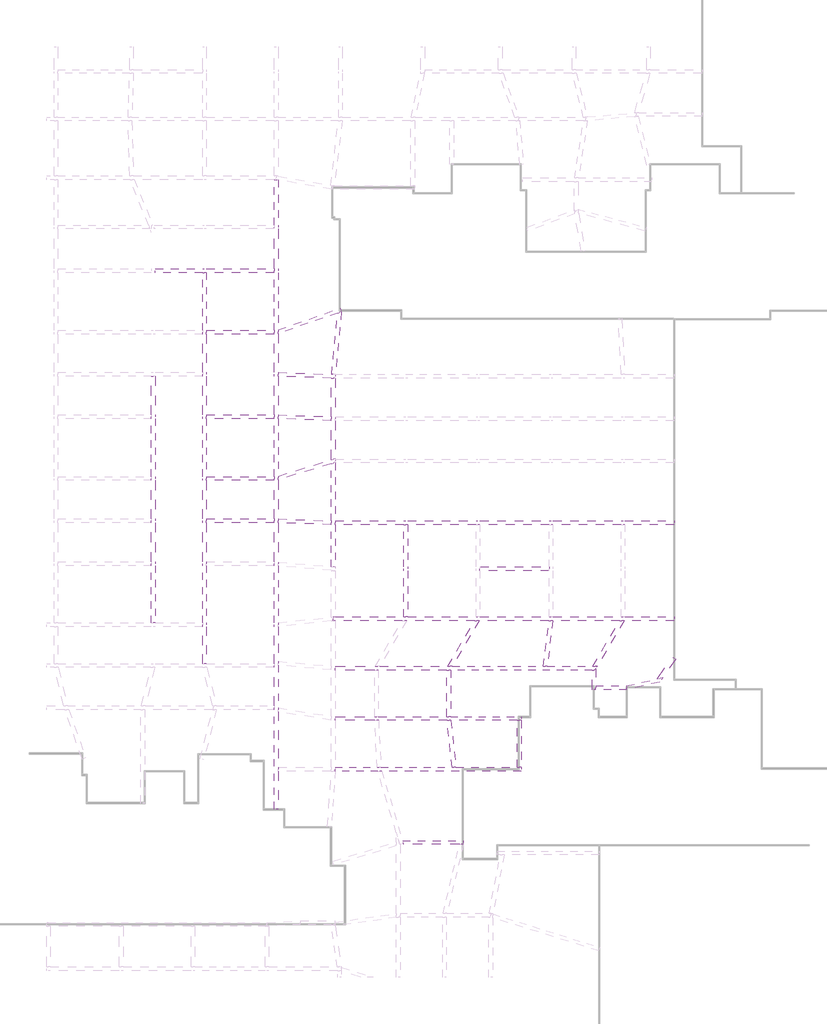
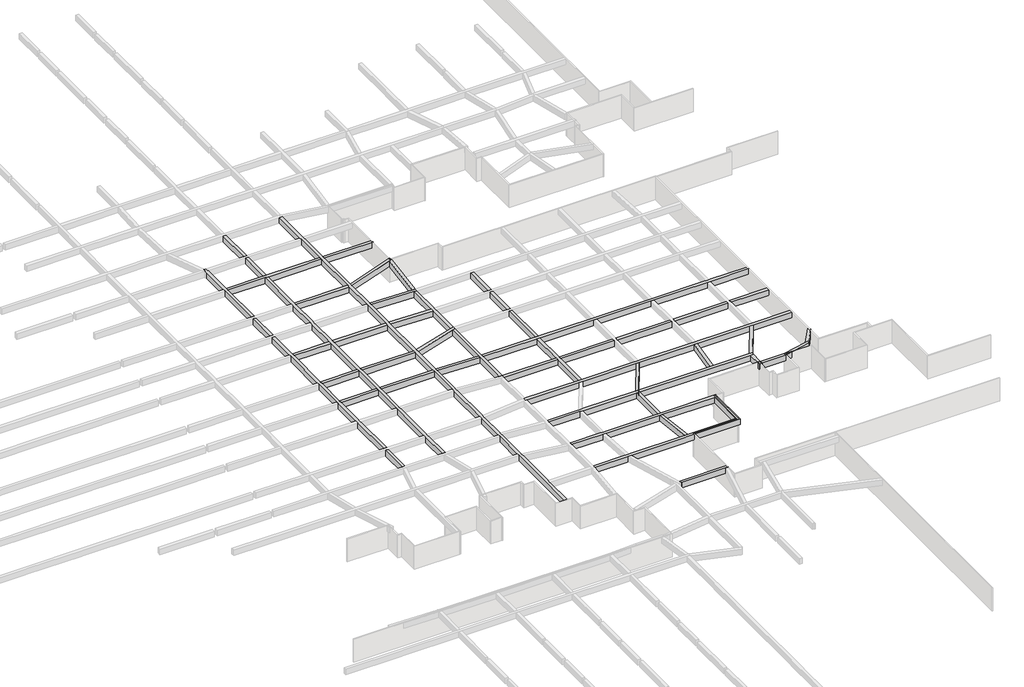
# One storey, part 42 of 45: 34 beams.
"""IFC4 building model written with IfcOpenShell, lengths in millimetres."""

import ifcopenshell
import ifcopenshell.guid

model = None  # the IFC model being written
_history = None  # IfcOwnerHistory: only IFC2X3 demands one
_inside = {}  # id of a spatial element -> (the spatial element, [elements in it])
_under = {}  # id of a project, library or spatial element -> (it, [spatial elements below it])
_declared = {}  # id of a project -> (the project, [libraries it declares])
_typed = {}  # id of a type object -> (the type object, [elements of that type])
_made_of = {}  # id of a material, layer set ... -> (it, [elements and type objects made of it])


def new_model(schema):
    """Start an empty IFC model of exactly this schema.

    Asked for "IFC4X3", IfcOpenShell would pick the latest addendum, in which some entities
    have other attributes; the version numbers below select the first issue.
    IFC2X3 requires an IfcOwnerHistory on every rooted entity: one is made here for all.
    """
    global model, _history
    if schema == "IFC4X3":
        model = ifcopenshell.file(schema_version=(4, 3, 0, 0))
    else:
        model = ifcopenshell.file(schema=schema)
    _inside.clear()
    _under.clear()
    _declared.clear()
    _typed.clear()
    _made_of.clear()
    _history = None
    if model.schema == "IFC2X3":
        org = make("IfcOrganization", Name="unknown")
        user = make(
            "IfcPersonAndOrganization",
            ThePerson=make("IfcPerson", FamilyName="unknown"),
            TheOrganization=org,
        )
        app = make(
            "IfcApplication",
            ApplicationDeveloper=org,
            Version="unknown",
            ApplicationFullName="unknown",
            ApplicationIdentifier="unknown",
        )
        _history = make(
            "IfcOwnerHistory",
            OwningUser=user,
            OwningApplication=app,
            ChangeAction="ADDED",
            CreationDate=0,
        )
    return model


def make(cls, **values):
    """One entity of the class cls with the attributes given. An attribute that is None is left unset."""
    return model.create_entity(
        cls, **{name: value for name, value in values.items() if value is not None}
    )


def rooted(cls, **values):
    """An entity with a GlobalId (a new one), such as an element, a storey or a relation."""
    return make(cls, GlobalId=ifcopenshell.guid.new(), OwnerHistory=_history, **values)


def si_unit(unit_type, name, prefix=None):
    """IfcSIUnit, for example si_unit("LENGTHUNIT", "METRE", prefix="MILLI")."""
    return make("IfcSIUnit", UnitType=unit_type, Prefix=prefix, Name=name)


def assignment(units):
    """IfcUnitAssignment: the units of a project."""
    return None if units is None else make("IfcUnitAssignment", Units=units)


def point(xyz):
    """IfcCartesianPoint."""
    return None if xyz is None else make("IfcCartesianPoint", Coordinates=xyz)


def direction(xyz):
    """IfcDirection."""
    return None if xyz is None else make("IfcDirection", DirectionRatios=xyz)


def frame(location, z_axis=None, x_axis=None):
    """IfcAxis2Placement3D, a coordinate frame: its origin and axes. An axis left out is left unset."""
    return make(
        "IfcAxis2Placement3D",
        Location=point(location),
        Axis=direction(z_axis),
        RefDirection=direction(x_axis),
    )


def origin():
    """The frame at (0, 0, 0) with its axes left unset."""
    return frame((0.0, 0.0, 0.0))


def place(relative_to, where):
    """IfcLocalPlacement: puts the frame where relative to a parent placement (None: the world)."""
    return make(
        "IfcLocalPlacement", PlacementRelTo=relative_to, RelativePlacement=where
    )


def context(
    kind, dimensions, precision=None, world=None, true_north=None, identifier=None
):
    """IfcGeometricRepresentationContext, for example the 3D "Model" context."""
    return make(
        "IfcGeometricRepresentationContext",
        ContextIdentifier=identifier,
        ContextType=kind,
        CoordinateSpaceDimension=dimensions,
        Precision=precision,
        WorldCoordinateSystem=world,
        TrueNorth=true_north,
    )


def project(units=None, contexts=None):
    """IfcProject with its units and contexts."""
    return rooted(
        "IfcProject",
        Name="project",
        RepresentationContexts=contexts,
        UnitsInContext=assignment(units),
    )


def spatial(cls, under=None, at=None, **own):
    """A site, building, storey or space (cls), placed at a placement, below another one or the project."""
    s = rooted(cls, ObjectPlacement=at, **own)
    if under is not None:
        _under.setdefault(under.id(), (under, []))[1].append(s)
    return s


def polyline(points):
    """IfcPolyline through the points."""
    return make("IfcPolyline", Points=[point(p) for p in points])


def outline(outer, holes=None, kind="AREA"):
    """IfcArbitraryClosedProfileDef: a profile drawn as a closed curve; with holes, ...WithVoids."""
    if holes is None:
        return make("IfcArbitraryClosedProfileDef", ProfileType=kind, OuterCurve=outer)
    return make(
        "IfcArbitraryProfileDefWithVoids",
        ProfileType=kind,
        OuterCurve=outer,
        InnerCurves=holes,
    )


def extrude(swept, where, along, depth):
    """IfcExtrudedAreaSolid: the profile swept, set in the frame where, extruded along a direction by depth."""
    return make(
        "IfcExtrudedAreaSolid",
        SweptArea=swept,
        Position=where,
        ExtrudedDirection=direction(along),
        Depth=depth,
    )


def faces_of(points, faces, orient=None, outer=None):
    """IfcFace entities. A face is a list of loops; a loop is a list of indices into points, from 0.

    orient and outer hold one flag for each loop. By default every Orientation is true, the
    first loop of a face is its IfcFaceOuterBound and the others are IfcFaceBound.
    """
    made = []
    for i, loops in enumerate(faces):
        bounds = []
        for j, loop in enumerate(loops):
            is_outer = j == 0 if outer is None else outer[i][j]
            bounds.append(
                make(
                    "IfcFaceOuterBound" if is_outer else "IfcFaceBound",
                    Bound=make("IfcPolyLoop", Polygon=[points[k] for k in loop]),
                    Orientation=True if orient is None else orient[i][j],
                )
            )
        made.append(make("IfcFace", Bounds=bounds))
    return made


def faceted_brep(points, faces, orient=None, outer=None, voids=None):
    """IfcFacetedBrep: a solid bounded by flat faces; with voids (closed shells), ...WithVoids."""
    shared = [point(p) for p in points]
    hull = make("IfcClosedShell", CfsFaces=faces_of(shared, faces, orient, outer))
    if voids is None:
        return make("IfcFacetedBrep", Outer=hull)
    return make(
        "IfcFacetedBrepWithVoids",
        Outer=hull,
        Voids=[
            make(cls, CfsFaces=faces_of(shared, fs, o, b)) for cls, fs, o, b in voids
        ],
    )


def shape(context_of_items, identifier, shape_type, items):
    """IfcShapeRepresentation: the items that make up one representation, for example the "Body"."""
    return make(
        "IfcShapeRepresentation",
        ContextOfItems=context_of_items,
        RepresentationIdentifier=identifier,
        RepresentationType=shape_type,
        Items=items,
    )


def made_of(thing, what):
    """Note that an element or type object is made of a material, layer set ...; save() writes the relation."""
    if what is not None:
        _made_of.setdefault(what.id(), (what, []))[1].append(thing)
    return thing


def element(
    cls,
    number,
    at=None,
    inside=None,
    cuts=None,
    type_object=None,
    material=None,
    context=None,
    identifier="Body",
    shape_type=None,
    held_by="IfcProductDefinitionShape",
    body=None,
    shapes=None,
    **own,
):
    """One element of the class cls, such as IfcWall. Its Tag is "e" and its number.

    at: its placement. inside: the storey or other place that contains it. cuts: it is an
    opening in that element (IfcRelVoidsElement). A single representation is given by context,
    identifier, shape_type and body (its items); several are given by shapes. held_by: the class
    of the entity that holds the representations. save() writes the other relations.
    """
    e = rooted(cls, Tag="e%d" % number, ObjectPlacement=at, **own)
    if body is not None:
        shapes = [shape(context, identifier, shape_type, body)]
    if shapes is not None:
        e.Representation = make(held_by, Representations=shapes)
    if inside is not None:
        _inside.setdefault(inside.id(), (inside, []))[1].append(e)
    if cuts is not None:
        rooted(
            "IfcRelVoidsElement", RelatingBuildingElement=cuts, RelatedOpeningElement=e
        )
    if type_object is not None:
        _typed.setdefault(type_object.id(), (type_object, []))[1].append(e)
    return made_of(e, material)


def aggregate(whole, parts):
    """IfcRelAggregates: a whole, such as a stair, and the parts it consists of."""
    return rooted("IfcRelAggregates", RelatingObject=whole, RelatedObjects=parts)


def save(model, path):
    """Write the relations noted so far, then the file.

    IfcRelAggregates (storeys below a building ...), IfcRelContainedInSpatialStructure (elements
    in a storey), IfcRelDefinesByType, IfcRelAssociatesMaterial and IfcRelDeclares: one each for
    every whole, place, type object, material and project.
    """
    for whole, parts in _under.values():
        aggregate(whole, parts)
    for where, things in _inside.values():
        rooted(
            "IfcRelContainedInSpatialStructure",
            RelatedElements=things,
            RelatingStructure=where,
        )
    for kind, things in _typed.values():
        rooted("IfcRelDefinesByType", RelatedObjects=things, RelatingType=kind)
    for what, things in _made_of.values():
        rooted("IfcRelAssociatesMaterial", RelatedObjects=things, RelatingMaterial=what)
    for by, libraries in _declared.values():
        rooted("IfcRelDeclares", RelatingContext=by, RelatedDefinitions=libraries)
    model.write(path)


model = new_model("IFC4")

# Units and contexts
model_context = context("Model", 3, world=origin())
ifc_project = project(units=[si_unit("LENGTHUNIT", "METRE", prefix="MILLI")], contexts=[model_context])

# Site, building, storey
site = spatial("IfcSite", under=ifc_project)
building = spatial("IfcBuilding", under=site)
storey = spatial("IfcBuildingStorey", under=building, Name="户型图", Elevation=0.0)

# Beams
placement = place(None, origin())
element("IfcBeam", 1, ObjectType="混凝土 - 矩形梁 : KL_beam", at=placement, inside=storey, context=model_context, shape_type="Brep", body=[
    faceted_brep([(18058.0309094, 68422.9728882, 3300.0), (17658.0309094, 68422.9728882, 3300.0), (17658.0309094, 68422.9728882, 2500.0), (18058.0309094, 68422.9728882, 2500.0), (18058.0309094, 72491.389713, 3300.0), (18058.0309094, 72891.389713, 3300.0), (18058.0309094, 78847.1860391, 3300.0), (18058.0309094, 79252.1720894, 3300.0), (18058.0309094, 83829.2308834, 3300.0), (18058.0309094, 84230.7588184, 3300.0), (18058.0309094, 87967.4136101, 3300.0), (18058.0309094, 88369.6169219, 3300.0), (18058.0309094, 94470.4509181, 3300.0), (18058.0309094, 94871.9788531, 3300.0), (18058.0309094, 99081.6059995, 3300.0), (18058.0309094, 99481.8498172, 3300.0), (18058.0309094, 103663.2536994, 3300.0), (18058.0309094, 104081.530402, 3300.0), (18058.0309094, 110222.8260342, 3300.0), (18058.0309094, 110623.0698519, 3300.0), (18058.0309094, 114764.7475323, 3300.0), (18058.0309094, 115164.99135, 3300.0), (18058.0309094, 119319.9005194, 3300.0), (18058.0309094, 119742.9487918, 3300.0), (18058.0309094, 125862.5591329, 3300.0), (18058.0309094, 126262.5591329, 3300.0), (18058.0309094, 130536.5288825, 3300.0), (18058.0309094, 130936.5288825, 3300.0), (18058.0309094, 135784.6345106, 3300.0), (17840.6731553, 135822.9605472, 3300.0), (17658.0309094, 135822.9605472, 3300.0), (17658.0309094, 130936.5288825, 3300.0), (17658.0309094, 130536.5288825, 3300.0), (17658.0309094, 126262.5591329, 3300.0), (17658.0309094, 125862.5591329, 3300.0), (17658.0309094, 119662.5591329, 3300.0), (17658.0309094, 119262.5591329, 3300.0), (17658.0309094, 115171.853595, 3300.0), (17658.0309094, 114771.853595, 3300.0), (17658.0309094, 110629.932653, 3300.0), (17658.0309094, 110229.932653, 3300.0), (17658.0309094, 104011.2459144, 3300.0), (17658.0309094, 103611.2459144, 3300.0), (17658.0309094, 99488.7126183, 3300.0), (17658.0309094, 99088.7126183, 3300.0), (17658.0309094, 94888.7126183, 3300.0), (17658.0309094, 94488.7126183, 3300.0), (17658.0309094, 88347.4925836, 3300.0), (17658.0309094, 87947.4925836, 3300.0), (17658.0309094, 83990.1370817, 3300.0), (17658.0309094, 83590.1370817, 3300.0), (17658.0309094, 79472.5341829, 3300.0), (17658.0309094, 79072.5341829, 3300.0), (17658.0309094, 135822.9605472, 2500.0), (17658.0309094, 130936.5288825, 2500.0), (17658.0309094, 130536.5288825, 2500.0), (17658.0309094, 126262.5591329, 2500.0), (17658.0309094, 125862.5591329, 2500.0), (17658.0309094, 119662.5591329, 2500.0), (17658.0309094, 119262.5591329, 2500.0), (17658.0309094, 115171.853595, 2500.0), (17658.0309094, 114771.853595, 2500.0), (17658.0309094, 110629.932653, 2500.0), (17658.0309094, 110229.932653, 2500.0), (17658.0309094, 104011.2459144, 2500.0), (17658.0309094, 103611.2459144, 2500.0), (17658.0309094, 99488.7126183, 2500.0), (17658.0309094, 99088.7126183, 2500.0), (17658.0309094, 94888.7126183, 2500.0), (17658.0309094, 94488.7126183, 2500.0), (17658.0309094, 88347.4925836, 2500.0), (17658.0309094, 87947.4925836, 2500.0), (17658.0309094, 83990.1370817, 2500.0), (17658.0309094, 83590.1370817, 2500.0), (17658.0309094, 79472.5341829, 2500.0), (17658.0309094, 79072.5341829, 2500.0), (17840.6731553, 135822.9605472, 2500.0), (18058.0309094, 135784.6345106, 2500.0), (18058.0309094, 130936.5288825, 2500.0), (18058.0309094, 130536.5288825, 2500.0), (18058.0309094, 126262.5591329, 2500.0), (18058.0309094, 125862.5591329, 2500.0), (18058.0309094, 119742.9487918, 2500.0), (18058.0309094, 119319.9005194, 2500.0), (18058.0309094, 115164.99135, 2500.0), (18058.0309094, 114764.7475323, 2500.0), (18058.0309094, 110623.0698519, 2500.0), (18058.0309094, 110222.8260342, 2500.0), (18058.0309094, 104081.530402, 2500.0), (18058.0309094, 103663.2536994, 2500.0), (18058.0309094, 99481.8498172, 2500.0), (18058.0309094, 99081.6059995, 2500.0), (18058.0309094, 94871.9788531, 2500.0), (18058.0309094, 94470.4509181, 2500.0), (18058.0309094, 88369.6169219, 2500.0), (18058.0309094, 87967.4136101, 2500.0), (18058.0309094, 84230.7588184, 2500.0), (18058.0309094, 83829.2308834, 2500.0), (18058.0309094, 79252.1720894, 2500.0), (18058.0309094, 78847.1860391, 2500.0), (18058.0309094, 72891.389713, 2500.0), (18058.0309094, 72491.389713, 2500.0)], [[[0, 1, 2, 3]], [[1, 0, 4, 5, 6, 7, 8, 9, 10, 11, 12, 13, 14, 15, 16, 17, 18, 19, 20, 21, 22, 23, 24, 25, 26, 27, 28, 29, 30, 31, 32, 33, 34, 35, 36, 37, 38, 39, 40, 41, 42, 43, 44, 45, 46, 47, 48, 49, 50, 51, 52]], [[2, 1, 52, 51, 50, 49, 48, 47, 46, 45, 44, 43, 42, 41, 40, 39, 38, 37, 36, 35, 34, 33, 32, 31, 30, 53, 54, 55, 56, 57, 58, 59, 60, 61, 62, 63, 64, 65, 66, 67, 68, 69, 70, 71, 72, 73, 74, 75]], [[3, 2, 75, 74, 73, 72, 71, 70, 69, 68, 67, 66, 65, 64, 63, 62, 61, 60, 59, 58, 57, 56, 55, 54, 53, 76, 77, 78, 79, 80, 81, 82, 83, 84, 85, 86, 87, 88, 89, 90, 91, 92, 93, 94, 95, 96, 97, 98, 99, 100, 101]], [[0, 3, 101, 100, 99, 98, 97, 96, 95, 94, 93, 92, 91, 90, 89, 88, 87, 86, 85, 84, 83, 82, 81, 80, 79, 78, 77, 28, 27, 26, 25, 24, 23, 22, 21, 20, 19, 18, 17, 16, 15, 14, 13, 12, 11, 10, 9, 8, 7, 6, 5, 4]], [[30, 29, 76, 53]], [[29, 28, 77, 76]]]),
])
element("IfcBeam", 2, ObjectType="混凝土 - 矩形梁 : KL_beam", at=placement, inside=storey, context=model_context, shape_type="Brep", body=[
    faceted_brep([(24715.3696453, 126262.5591329, 3300.0), (24715.3696453, 125862.5591329, 3300.0), (24715.3696453, 125862.5591329, 2500.0), (24715.3696453, 126262.5591329, 2500.0), (18058.0309094, 126262.5591329, 3300.0), (18058.0309094, 125862.5591329, 3300.0), (18058.0309094, 125862.5591329, 2500.0), (18058.0309094, 126262.5591329, 2500.0)], [[[0, 1, 2, 3]], [[1, 0, 4, 5]], [[2, 1, 5, 6]], [[3, 2, 6, 7]], [[0, 3, 7, 4]], [[5, 4, 7, 6]]]),
    faceted_brep([(17658.0309094, 126262.5591329, 3300.0), (17658.0309094, 125862.5591329, 3300.0), (17658.0309094, 125862.5591329, 2500.0), (17658.0309094, 126262.5591329, 2500.0), (10373.3027926, 126262.5591329, 3300.0), (9973.3027926, 126262.5591329, 3300.0), (4900.9990644, 126262.5591329, 3300.0), (4900.9990644, 125862.5591329, 3300.0), (9973.3027926, 125862.5591329, 3300.0), (10373.3027926, 125862.5591329, 3300.0), (4900.9990644, 125862.5591329, 2500.0), (9973.3027926, 125862.5591329, 2500.0), (10373.3027926, 125862.5591329, 2500.0), (4900.9990644, 126262.5591329, 2500.0), (9973.3027926, 126262.5591329, 2500.0), (10373.3027926, 126262.5591329, 2500.0)], [[[0, 1, 2, 3]], [[1, 0, 4, 5, 6, 7, 8, 9]], [[2, 1, 9, 8, 7, 10, 11, 12]], [[3, 2, 12, 11, 10, 13, 14, 15]], [[0, 3, 15, 14, 13, 6, 5, 4]], [[7, 6, 13, 10]]]),
])
element("IfcBeam", 3, ObjectType="混凝土 - 矩形梁 : KL_beam", at=placement, inside=storey, context=model_context, shape_type="Brep", body=[
    faceted_brep([(10373.3027926, 135822.9605472, 3300.0), (9973.3027926, 135822.9605472, 3300.0), (9973.3027926, 130936.5288825, 3300.0), (10373.3027926, 130936.5288825, 3300.0), (9973.3027926, 135822.9605472, 2500.0), (9973.3027926, 130936.5288825, 2500.0), (10373.3027926, 135822.9605472, 2500.0), (10373.3027926, 130936.5288825, 2500.0)], [[[0, 1, 2, 3]], [[1, 4, 5, 2]], [[4, 6, 7, 5]], [[6, 0, 3, 7]], [[1, 0, 6, 4]], [[3, 2, 5, 7]]]),
    faceted_brep([(9973.3027926, 130536.5288825, 3300.0), (10373.3027926, 130536.5288825, 3300.0), (10373.3027926, 130536.5288825, 2500.0), (9973.3027926, 130536.5288825, 2500.0), (10373.3027926, 126262.5591329, 3300.0), (9973.3027926, 126262.5591329, 3300.0), (9973.3027926, 126262.5591329, 2500.0), (10373.3027926, 126262.5591329, 2500.0)], [[[0, 1, 2, 3]], [[4, 5, 6, 7]], [[1, 0, 5, 4]], [[0, 3, 6, 5]], [[3, 2, 7, 6]], [[2, 1, 4, 7]]]),
    faceted_brep([(10373.3027926, 125862.5591329, 3300.0), (9973.3027926, 125862.5591329, 3300.0), (9973.3027926, 119662.5591329, 3300.0), (9973.3027926, 119262.5591329, 3300.0), (9973.3027926, 115171.853595, 3300.0), (9973.3027926, 114771.853595, 3300.0), (9973.3027926, 110629.932653, 3300.0), (9973.3027926, 110229.932653, 3300.0), (9973.3027926, 104011.2459144, 3300.0), (9973.3027926, 103611.2459144, 3300.0), (9973.3027926, 99488.7126183, 3300.0), (9973.3027926, 99088.7126183, 3300.0), (9973.3027926, 94888.7126183, 3300.0), (9973.3027926, 94488.7126183, 3300.0), (9973.3027926, 88347.4925836, 3300.0), (9973.3027926, 87947.4925836, 3300.0), (9973.3027926, 83990.1370817, 3300.0), (10373.3027926, 83990.1370817, 3300.0), (10373.3027926, 87947.4925836, 3300.0), (10373.3027926, 88347.4925836, 3300.0), (10373.3027926, 94488.7126183, 3300.0), (10373.3027926, 94888.7126183, 3300.0), (10373.3027926, 99088.7126183, 3300.0), (10373.3027926, 99488.7126183, 3300.0), (10373.3027926, 103611.2459144, 3300.0), (10373.3027926, 104011.2459144, 3300.0), (10373.3027926, 110229.932653, 3300.0), (10373.3027926, 110629.932653, 3300.0), (10373.3027926, 114771.853595, 3300.0), (10373.3027926, 115171.853595, 3300.0), (10373.3027926, 119262.5591329, 3300.0), (10373.3027926, 119662.5591329, 3300.0), (9973.3027926, 125862.5591329, 2500.0), (9973.3027926, 119662.5591329, 2500.0), (9973.3027926, 119262.5591329, 2500.0), (9973.3027926, 115171.853595, 2500.0), (9973.3027926, 114771.853595, 2500.0), (9973.3027926, 110629.932653, 2500.0), (9973.3027926, 110229.932653, 2500.0), (9973.3027926, 104011.2459144, 2500.0), (9973.3027926, 103611.2459144, 2500.0), (9973.3027926, 99488.7126183, 2500.0), (9973.3027926, 99088.7126183, 2500.0), (9973.3027926, 94888.7126183, 2500.0), (9973.3027926, 94488.7126183, 2500.0), (9973.3027926, 88347.4925836, 2500.0), (9973.3027926, 87947.4925836, 2500.0), (9973.3027926, 83990.1370817, 2500.0), (10373.3027926, 125862.5591329, 2500.0), (10373.3027926, 119662.5591329, 2500.0), (10373.3027926, 119262.5591329, 2500.0), (10373.3027926, 115171.853595, 2500.0), (10373.3027926, 114771.853595, 2500.0), (10373.3027926, 110629.932653, 2500.0), (10373.3027926, 110229.932653, 2500.0), (10373.3027926, 104011.2459144, 2500.0), (10373.3027926, 103611.2459144, 2500.0), (10373.3027926, 99488.7126183, 2500.0), (10373.3027926, 99088.7126183, 2500.0), (10373.3027926, 94888.7126183, 2500.0), (10373.3027926, 94488.7126183, 2500.0), (10373.3027926, 88347.4925836, 2500.0), (10373.3027926, 87947.4925836, 2500.0), (10373.3027926, 83990.1370817, 2500.0)], [[[0, 1, 2, 3, 4, 5, 6, 7, 8, 9, 10, 11, 12, 13, 14, 15, 16, 17, 18, 19, 20, 21, 22, 23, 24, 25, 26, 27, 28, 29, 30, 31]], [[1, 32, 33, 34, 35, 36, 37, 38, 39, 40, 41, 42, 43, 44, 45, 46, 47, 16, 15, 14, 13, 12, 11, 10, 9, 8, 7, 6, 5, 4, 3, 2]], [[32, 48, 49, 50, 51, 52, 53, 54, 55, 56, 57, 58, 59, 60, 61, 62, 63, 47, 46, 45, 44, 43, 42, 41, 40, 39, 38, 37, 36, 35, 34, 33]], [[48, 0, 31, 30, 29, 28, 27, 26, 25, 24, 23, 22, 21, 20, 19, 18, 17, 63, 62, 61, 60, 59, 58, 57, 56, 55, 54, 53, 52, 51, 50, 49]], [[1, 0, 48, 32]], [[17, 16, 47, 63]]]),
])
element("IfcBeam", 4, ObjectType="混凝土 - 矩形梁 : KL_beam", at=placement, inside=storey, context=model_context, shape_type="SweptSolid", body=[
    extrude(outline(polyline([(17658.0309094, 119662.5591329), (17658.0309094, 119262.5591329), (10373.3027926, 119262.5591329), (10373.3027926, 119662.5591329), (17658.0309094, 119662.5591329)])), frame((0.0, 0.0, 2500.0), z_axis=(0.0, 0.0, 1.0), x_axis=(1.0, 0.0, 0.0)), (0.0, 0.0, 1.0), 800.0),
])
element("IfcBeam", 5, ObjectType="混凝土 - 矩形梁 : KL_beam", at=placement, inside=storey, context=model_context, shape_type="Brep", body=[
    faceted_brep([(24852.3513635, 121659.3726652, 3300.0), (24722.1241017, 122037.5800955, 3300.0), (18058.0309094, 119742.9487918, 3300.0), (18058.0309094, 119319.9005194, 3300.0), (24436.4902984, 121516.1802172, 3300.0), (24852.3513635, 121659.3726652, 2500.0), (18058.0309094, 119319.9005194, 2500.0), (24436.4902984, 121516.1802172, 2500.0), (24722.1241017, 122037.5800955, 2500.0), (18058.0309094, 119742.9487918, 2500.0)], [[[0, 1, 2, 3, 4]], [[5, 0, 4, 3, 6, 7]], [[8, 5, 7, 6, 9]], [[1, 8, 9, 2]], [[3, 2, 9, 6]], [[1, 0, 5, 8]]]),
])
element("IfcBeam", 6, ObjectType="混凝土 - 矩形梁 : KL_beam", at=placement, inside=storey, context=model_context, shape_type="SweptSolid", body=[
    extrude(outline(polyline([(4900.9990644, 99088.7126183), (4900.9990644, 99488.7126183), (9973.3027926, 99488.7126183), (9973.3027926, 99088.7126183), (4900.9990644, 99088.7126183)])), frame((0.0, 0.0, 2500.0), z_axis=(0.0, 0.0, 1.0), x_axis=(1.0, 0.0, 0.0)), (0.0, 0.0, 1.0), 800.0),
    extrude(outline(polyline([(17658.0309094, 99488.7126183), (17658.0309094, 99088.7126183), (10373.3027926, 99088.7126183), (10373.3027926, 99488.7126183), (17658.0309094, 99488.7126183)])), frame((0.0, 0.0, 2500.0), z_axis=(0.0, 0.0, 1.0), x_axis=(1.0, 0.0, 0.0)), (0.0, 0.0, 1.0), 800.0),
])
element("IfcBeam", 7, ObjectType="混凝土 - 矩形梁 : KL_beam", at=placement, inside=storey, context=model_context, shape_type="SweptSolid", body=[
    extrude(outline(polyline([(4900.9990644, 103611.2459144), (4900.9990644, 104011.2459144), (9973.3027926, 104011.2459144), (9973.3027926, 103611.2459144), (4900.9990644, 103611.2459144)])), frame((0.0, 0.0, 2500.0), z_axis=(0.0, 0.0, 1.0), x_axis=(1.0, 0.0, 0.0)), (0.0, 0.0, 1.0), 800.0),
    extrude(outline(polyline([(17658.0309094, 104011.2459144), (17658.0309094, 103611.2459144), (10373.3027926, 103611.2459144), (10373.3027926, 104011.2459144), (17658.0309094, 104011.2459144)])), frame((0.0, 0.0, 2500.0), z_axis=(0.0, 0.0, 1.0), x_axis=(1.0, 0.0, 0.0)), (0.0, 0.0, 1.0), 800.0),
])
element("IfcBeam", 8, ObjectType="混凝土 - 矩形梁 : KL_beam", at=placement, inside=storey, context=model_context, shape_type="SweptSolid", body=[
    extrude(outline(polyline([(4900.9990644, 110229.932653), (4900.9990644, 110629.932653), (9973.3027926, 110629.932653), (9973.3027926, 110229.932653), (4900.9990644, 110229.932653)])), frame((0.0, 0.0, 2500.0), z_axis=(0.0, 0.0, 1.0), x_axis=(1.0, 0.0, 0.0)), (0.0, 0.0, 1.0), 800.0),
    extrude(outline(polyline([(17658.0309094, 110629.932653), (17658.0309094, 110229.932653), (10373.3027926, 110229.932653), (10373.3027926, 110629.932653), (17658.0309094, 110629.932653)])), frame((0.0, 0.0, 2500.0), z_axis=(0.0, 0.0, 1.0), x_axis=(1.0, 0.0, 0.0)), (0.0, 0.0, 1.0), 800.0),
])
element("IfcBeam", 9, ObjectType="混凝土 - 矩形梁 : KL_beam", at=placement, inside=storey, context=model_context, shape_type="Brep", body=[
    faceted_brep([(4900.9990644, 130536.5288825, 3300.0), (4809.3709906, 130536.5288825, 3300.0), (4809.3709906, 130936.5288825, 3300.0), (4635.6642065, 130936.5288825, 3300.0), (4500.9990644, 130936.5288825, 3300.0), (4500.9990644, 130199.5727008, 3300.0), (4500.9990644, 126262.5591329, 3300.0), (4500.9990644, 125862.5591329, 3300.0), (4500.9990644, 119662.5591329, 3300.0), (4900.9990644, 119662.5591329, 3300.0), (4900.9990644, 125862.5591329, 3300.0), (4900.9990644, 126262.5591329, 3300.0), (4500.9990644, 119662.5591329, 2500.0), (4500.9990644, 130936.5288825, 2500.0), (4500.9990644, 130199.5727008, 2500.0), (4500.9990644, 126262.5591329, 2500.0), (4500.9990644, 125862.5591329, 2500.0), (4809.3709906, 130536.5288825, 2500.0), (4900.9990644, 130536.5288825, 2500.0), (4900.9990644, 126262.5591329, 2500.0), (4900.9990644, 125862.5591329, 2500.0), (4900.9990644, 119662.5591329, 2500.0), (4635.6642065, 130936.5288825, 2500.0), (4809.3709906, 130936.5288825, 2500.0)], [[[0, 1, 2, 3, 4, 5, 6, 7, 8, 9, 10, 11]], [[12, 8, 7, 6, 5, 4, 13, 14, 15, 16]], [[17, 18, 19, 20, 21, 12, 16, 15, 14, 13, 22, 23]], [[18, 0, 11, 10, 9, 21, 20, 19]], [[1, 0, 18, 17]], [[9, 8, 12, 21]], [[1, 17, 23, 2]], [[13, 4, 3, 2, 23, 22]]]),
    faceted_brep([(4500.9990644, 119262.5591329, 3300.0), (4900.9990644, 119262.5591329, 3300.0), (4900.9990644, 119262.5591329, 2500.0), (4500.9990644, 119262.5591329, 2500.0), (4900.9990644, 115171.853595, 3300.0), (4500.9990644, 115171.853595, 3300.0), (4500.9990644, 115171.853595, 2500.0), (4900.9990644, 115171.853595, 2500.0)], [[[0, 1, 2, 3]], [[4, 5, 6, 7]], [[1, 0, 5, 4]], [[0, 3, 6, 5]], [[3, 2, 7, 6]], [[2, 1, 4, 7]]]),
    faceted_brep([(4900.9990644, 114771.853595, 3300.0), (4500.9990644, 114771.853595, 3300.0), (4500.9990644, 110629.932653, 3300.0), (4500.9990644, 110229.932653, 3300.0), (4500.9990644, 104011.2459144, 3300.0), (4500.9990644, 103611.2459144, 3300.0), (4500.9990644, 99488.7126183, 3300.0), (4500.9990644, 99088.7126183, 3300.0), (4500.9990644, 94888.7126183, 3300.0), (4500.9990644, 94488.7126183, 3300.0), (4500.9990644, 88347.4925836, 3300.0), (4900.9990644, 88347.4925836, 3300.0), (4900.9990644, 94488.7126183, 3300.0), (4900.9990644, 94888.7126183, 3300.0), (4900.9990644, 99088.7126183, 3300.0), (4900.9990644, 99488.7126183, 3300.0), (4900.9990644, 103611.2459144, 3300.0), (4900.9990644, 104011.2459144, 3300.0), (4900.9990644, 110229.932653, 3300.0), (4900.9990644, 110629.932653, 3300.0), (4500.9990644, 114771.853595, 2500.0), (4500.9990644, 110629.932653, 2500.0), (4500.9990644, 110229.932653, 2500.0), (4500.9990644, 104011.2459144, 2500.0), (4500.9990644, 103611.2459144, 2500.0), (4500.9990644, 99488.7126183, 2500.0), (4500.9990644, 99088.7126183, 2500.0), (4500.9990644, 94888.7126183, 2500.0), (4500.9990644, 94488.7126183, 2500.0), (4500.9990644, 88347.4925836, 2500.0), (4900.9990644, 114771.853595, 2500.0), (4900.9990644, 110629.932653, 2500.0), (4900.9990644, 110229.932653, 2500.0), (4900.9990644, 104011.2459144, 2500.0), (4900.9990644, 103611.2459144, 2500.0), (4900.9990644, 99488.7126183, 2500.0), (4900.9990644, 99088.7126183, 2500.0), (4900.9990644, 94888.7126183, 2500.0), (4900.9990644, 94488.7126183, 2500.0), (4900.9990644, 88347.4925836, 2500.0)], [[[0, 1, 2, 3, 4, 5, 6, 7, 8, 9, 10, 11, 12, 13, 14, 15, 16, 17, 18, 19]], [[1, 20, 21, 22, 23, 24, 25, 26, 27, 28, 29, 10, 9, 8, 7, 6, 5, 4, 3, 2]], [[20, 30, 31, 32, 33, 34, 35, 36, 37, 38, 39, 29, 28, 27, 26, 25, 24, 23, 22, 21]], [[30, 0, 19, 18, 17, 16, 15, 14, 13, 12, 11, 39, 38, 37, 36, 35, 34, 33, 32, 31]], [[1, 0, 30, 20]], [[11, 10, 29, 39]]]),
    faceted_brep([(4500.9990644, 87947.4925836, 3300.0), (4900.9990644, 87947.4925836, 3300.0), (4900.9990644, 87947.4925836, 2500.0), (4500.9990644, 87947.4925836, 2500.0), (4500.9990644, 83990.1370817, 3300.0), (4900.9990644, 83990.1370817, 3300.0), (4500.9990644, 83990.1370817, 2500.0), (4900.9990644, 83990.1370817, 2500.0)], [[[0, 1, 2, 3]], [[1, 0, 4, 5]], [[0, 3, 6, 4]], [[3, 2, 7, 6]], [[2, 1, 5, 7]], [[5, 4, 6, 7]]]),
])
element("IfcBeam", 10, ObjectType="混凝土 - 矩形梁 : KL_beam", at=placement, inside=storey, context=model_context, shape_type="Brep", body=[
    faceted_brep([(24178.3813476, 114551.0201854, 3300.0), (24178.3813476, 114558.1276627, 3300.0), (24178.3813476, 114951.2640031, 3300.0), (23981.8318538, 114958.1276627, 3300.0), (23797.5977176, 114964.5612605, 3300.0), (18058.0309094, 115164.99135, 3300.0), (18058.0309094, 114764.7475323, 3300.0), (23778.3813476, 114564.9884932, 3300.0), (24178.3813476, 114551.0201854, 2500.0), (18058.0309094, 114764.7475323, 2500.0), (23778.3813476, 114564.9884932, 2500.0), (24178.3813476, 114951.2640031, 2500.0), (24178.3813476, 114558.1276627, 2500.0), (18058.0309094, 115164.99135, 2500.0), (23797.5977176, 114964.5612605, 2500.0), (23981.8318538, 114958.1276627, 2500.0)], [[[0, 1, 2, 3, 4, 5, 6, 7]], [[8, 0, 7, 6, 9, 10]], [[11, 12, 8, 10, 9, 13, 14, 15]], [[2, 11, 15, 14, 13, 5, 4, 3]], [[6, 5, 13, 9]], [[2, 1, 0, 8, 12, 11]]]),
])
element("IfcBeam", 11, ObjectType="混凝土 - 矩形梁 : KL_beam", at=placement, inside=storey, context=model_context, shape_type="SweptSolid", body=[
    extrude(outline(polyline([(18058.0309094, 110222.8260342), (18058.0309094, 110623.0698519), (23778.3813476, 110423.3108128), (23778.3813476, 110023.0669951), (18058.0309094, 110222.8260342)])), frame((0.0, 0.0, 2500.0), z_axis=(0.0, 0.0, 1.0), x_axis=(1.0, 0.0, 0.0)), (0.0, 0.0, 1.0), 800.0),
])
element("IfcBeam", 12, ObjectType="混凝土 - 矩形梁 : KL_beam", at=placement, inside=storey, context=model_context, shape_type="Brep", body=[
    faceted_brep([(24178.3813476, 105534.4326096, 3300.0), (24178.3813476, 105882.8380814, 3300.0), (24178.3813476, 105952.7093122, 3300.0), (23778.3813476, 105830.4170396, 3300.0), (18058.0309094, 104081.530402, 3300.0), (18058.0309094, 103663.2536994, 3300.0), (23778.3813476, 105412.140337, 3300.0), (24178.3813476, 105534.4326096, 2500.0), (18058.0309094, 103663.2536994, 2500.0), (23778.3813476, 105412.140337, 2500.0), (24178.3813476, 105952.7093122, 2500.0), (24178.3813476, 105882.8380814, 2500.0), (18058.0309094, 104081.530402, 2500.0), (23778.3813476, 105830.4170396, 2500.0)], [[[0, 1, 2, 3, 4, 5, 6]], [[7, 0, 6, 5, 8, 9]], [[10, 11, 7, 9, 8, 12, 13]], [[2, 10, 13, 12, 4, 3]], [[5, 4, 12, 8]], [[2, 1, 0, 7, 11, 10]]]),
])
element("IfcBeam", 13, ObjectType="混凝土 - 矩形梁 : KL_beam", at=placement, inside=storey, context=model_context, shape_type="Brep", body=[
    faceted_brep([(24178.3813476, 114551.0201854, 3300.0), (23778.3813476, 114564.9884932, 3300.0), (23778.3813476, 110423.3108128, 3300.0), (23778.3813476, 110023.0669951, 3300.0), (23778.3813476, 105830.4170396, 3300.0), (24178.3813476, 105952.7093122, 3300.0), (24178.3813476, 110016.1887149, 3300.0), (24178.3813476, 110416.1887149, 3300.0), (24178.3813476, 114551.0201854, 2500.0), (24178.3813476, 105952.7093122, 2500.0), (24178.3813476, 110016.1887149, 2500.0), (24178.3813476, 110416.1887149, 2500.0), (23778.3813476, 114564.9884932, 2500.0), (23778.3813476, 105830.4170396, 2500.0), (23778.3813476, 110023.0669951, 2500.0), (23778.3813476, 110423.3108128, 2500.0)], [[[0, 1, 2, 3, 4, 5, 6, 7]], [[8, 0, 7, 6, 5, 9, 10, 11]], [[12, 8, 11, 10, 9, 13, 14, 15]], [[1, 12, 15, 14, 13, 4, 3, 2]], [[1, 0, 8, 12]], [[5, 4, 13, 9]]]),
])
element("IfcBeam", 14, ObjectType="混凝土 - 矩形梁 : KL_beam", at=placement, inside=storey, context=model_context, shape_type="SweptSolid", body=[
    extrude(outline(polyline([(18058.0309094, 99081.6059995), (18058.0309094, 99481.8498172), (23778.3813476, 99282.0907782), (23778.3813476, 98881.8469604), (18058.0309094, 99081.6059995)])), frame((0.0, 0.0, 2500.0), z_axis=(0.0, 0.0, 1.0), x_axis=(1.0, 0.0, 0.0)), (0.0, 0.0, 1.0), 800.0),
])
element("IfcBeam", 15, ObjectType="混凝土 - 矩形梁 : KL_beam", at=placement, inside=storey, context=model_context, shape_type="Brep", body=[
    faceted_brep([(24178.3813476, 94336.517573, 3300.0), (24178.3813476, 94353.2831144, 3300.0), (24178.3813476, 98874.9847154, 3300.0), (24178.3813476, 99274.9847154, 3300.0), (24178.3813476, 105482.8380814, 3300.0), (24178.3813476, 105534.4326096, 3300.0), (23778.3813476, 105412.140337, 3300.0), (23778.3813476, 99282.0907782, 3300.0), (23778.3813476, 98881.8469604, 3300.0), (23778.3813476, 94371.5130384, 3300.0), (24178.3813476, 94336.517573, 2500.0), (24178.3813476, 94353.2831144, 2500.0), (24178.3813476, 98874.9847154, 2500.0), (24178.3813476, 99274.9847154, 2500.0), (24178.3813476, 105482.8380814, 2500.0), (24178.3813476, 105534.4326096, 2500.0), (23778.3813476, 94371.5130384, 2500.0), (23778.3813476, 98881.8469604, 2500.0), (23778.3813476, 99282.0907782, 2500.0), (23778.3813476, 105412.140337, 2500.0)], [[[0, 1, 2, 3, 4, 5, 6, 7, 8, 9]], [[5, 4, 3, 2, 1, 0, 10, 11, 12, 13, 14, 15]], [[15, 14, 13, 12, 11, 10, 16, 17, 18, 19]], [[6, 19, 18, 17, 16, 9, 8, 7]], [[6, 5, 15, 19]], [[0, 9, 16, 10]]]),
])
element("IfcBeam", 16, ObjectType="混凝土 - 矩形梁 : KL_beam", at=placement, inside=storey, context=model_context, shape_type="Brep", body=[
    faceted_brep([(60459.4298456, 99274.9847154, 3300.0), (60459.4298456, 98874.9847154, 3300.0), (60459.4298456, 98874.9847154, 2500.0), (60459.4298456, 99274.9847154, 2500.0), (55199.4783436, 99274.9847154, 3300.0), (54799.4783436, 99274.9847154, 3300.0), (47494.6087163, 99274.9847154, 3300.0), (47094.6087163, 99274.9847154, 3300.0), (39666.3635798, 99274.9847154, 3300.0), (39266.3635798, 99274.9847154, 3300.0), (31925.9205959, 99274.9847154, 3300.0), (31525.9205959, 99274.9847154, 3300.0), (24178.3813476, 99274.9847154, 3300.0), (24178.3813476, 98874.9847154, 3300.0), (31525.9205959, 98874.9847154, 3300.0), (31925.9205959, 98874.9847154, 3300.0), (39266.3635798, 98874.9847154, 3300.0), (39666.3635798, 98874.9847154, 3300.0), (47094.6087163, 98874.9847154, 3300.0), (47494.6087163, 98874.9847154, 3300.0), (54799.4783436, 98874.9847154, 3300.0), (55199.4783436, 98874.9847154, 3300.0), (24178.3813476, 98874.9847154, 2500.0), (31525.9205959, 98874.9847154, 2500.0), (31925.9205959, 98874.9847154, 2500.0), (39266.3635798, 98874.9847154, 2500.0), (39666.3635798, 98874.9847154, 2500.0), (47094.6087163, 98874.9847154, 2500.0), (47494.6087163, 98874.9847154, 2500.0), (54799.4783436, 98874.9847154, 2500.0), (55199.4783436, 98874.9847154, 2500.0), (24178.3813476, 99274.9847154, 2500.0), (31525.9205959, 99274.9847154, 2500.0), (31925.9205959, 99274.9847154, 2500.0), (39266.3635798, 99274.9847154, 2500.0), (39666.3635798, 99274.9847154, 2500.0), (47094.6087163, 99274.9847154, 2500.0), (47494.6087163, 99274.9847154, 2500.0), (54799.4783436, 99274.9847154, 2500.0), (55199.4783436, 99274.9847154, 2500.0)], [[[0, 1, 2, 3]], [[1, 0, 4, 5, 6, 7, 8, 9, 10, 11, 12, 13, 14, 15, 16, 17, 18, 19, 20, 21]], [[2, 1, 21, 20, 19, 18, 17, 16, 15, 14, 13, 22, 23, 24, 25, 26, 27, 28, 29, 30]], [[3, 2, 30, 29, 28, 27, 26, 25, 24, 23, 22, 31, 32, 33, 34, 35, 36, 37, 38, 39]], [[0, 3, 39, 38, 37, 36, 35, 34, 33, 32, 31, 12, 11, 10, 9, 8, 7, 6, 5, 4]], [[13, 12, 31, 22]]]),
])
element("IfcBeam", 17, ObjectType="混凝土 - 矩形梁 : KL_beam", at=placement, inside=storey, context=model_context, shape_type="SweptSolid", body=[
    extrude(outline(polyline([(24436.4902984, 121516.1802172), (24852.3513635, 121659.3726652), (24198.8677371, 114958.1276627), (23981.8318538, 114958.1276627), (23797.5977176, 114964.5612605), (24436.4902984, 121516.1802172)])), frame((0.0, 0.0, 2500.0), z_axis=(0.0, 0.0, 1.0), x_axis=(1.0, 0.0, 0.0)), (0.0, 0.0, 1.0), 800.0),
])
element("IfcBeam", 18, ObjectType="混凝土 - 矩形梁 : KL_beam", at=placement, inside=storey, context=model_context, shape_type="Brep", body=[
    faceted_brep([(31925.9205959, 114558.1276627, 3300.0), (31525.9205959, 114558.1276627, 3300.0), (31525.9205959, 110416.1887149, 3300.0), (31925.9205959, 110416.1887149, 3300.0), (31525.9205959, 114558.1276627, 2500.0), (31525.9205959, 110416.1887149, 2500.0), (31925.9205959, 114558.1276627, 2500.0), (31925.9205959, 110416.1887149, 2500.0)], [[[0, 1, 2, 3]], [[1, 4, 5, 2]], [[4, 6, 7, 5]], [[6, 0, 3, 7]], [[1, 0, 6, 4]], [[3, 2, 5, 7]]]),
    faceted_brep([(31525.9205959, 98874.9847154, 3300.0), (31925.9205959, 98874.9847154, 3300.0), (31925.9205959, 98874.9847154, 2500.0), (31525.9205959, 98874.9847154, 2500.0), (31525.9205959, 94353.2831144, 3300.0), (31525.9205959, 93953.2831144, 3300.0), (31525.9205959, 88990.7691713, 3300.0), (31925.9205959, 88990.7691713, 3300.0), (31925.9205959, 93953.2831144, 3300.0), (31925.9205959, 94353.2831144, 3300.0), (31525.9205959, 94353.2831144, 2500.0), (31525.9205959, 93953.2831144, 2500.0), (31525.9205959, 88990.7691713, 2500.0), (31925.9205959, 94353.2831144, 2500.0), (31925.9205959, 93953.2831144, 2500.0), (31925.9205959, 88990.7691713, 2500.0)], [[[0, 1, 2, 3]], [[1, 0, 4, 5, 6, 7, 8, 9]], [[0, 3, 10, 11, 12, 6, 5, 4]], [[3, 2, 13, 14, 15, 12, 11, 10]], [[2, 1, 9, 8, 7, 15, 14, 13]], [[7, 6, 12, 15]]]),
    faceted_brep([(31925.9205959, 99274.9847154, 3300.0), (31525.9205959, 99274.9847154, 3300.0), (31525.9205959, 99274.9847154, 2500.0), (31925.9205959, 99274.9847154, 2500.0), (31525.9205959, 105482.8380814, 3300.0), (31925.9205959, 105482.8380814, 3300.0), (31925.9205959, 105482.8380814, 2500.0), (31525.9205959, 105482.8380814, 2500.0)], [[[0, 1, 2, 3]], [[4, 5, 6, 7]], [[1, 0, 5, 4]], [[2, 1, 4, 7]], [[3, 2, 7, 6]], [[0, 3, 6, 5]]]),
    faceted_brep([(31925.9205959, 105882.8380814, 3300.0), (31525.9205959, 105882.8380814, 3300.0), (31525.9205959, 105882.8380814, 2500.0), (31925.9205959, 105882.8380814, 2500.0), (31525.9205959, 110016.1887149, 3300.0), (31925.9205959, 110016.1887149, 3300.0), (31925.9205959, 110016.1887149, 2500.0), (31525.9205959, 110016.1887149, 2500.0)], [[[0, 1, 2, 3]], [[4, 5, 6, 7]], [[1, 0, 5, 4]], [[2, 1, 4, 7]], [[3, 2, 7, 6]], [[0, 3, 6, 5]]]),
])
element("IfcBeam", 19, ObjectType="混凝土 - 矩形梁 : KL_beam", at=placement, inside=storey, context=model_context, shape_type="Brep", body=[
    faceted_brep([(60459.4298456, 94353.2831144, 3300.0), (60459.4298456, 93953.2831144, 3300.0), (60459.4298456, 93953.2831144, 2500.0), (60459.4298456, 94353.2831144, 2500.0), (55199.4783436, 94353.2831144, 3300.0), (55199.4783436, 93953.2831144, 3300.0), (55199.4783436, 93953.2831144, 2500.0), (55199.4783436, 94353.2831144, 2500.0)], [[[0, 1, 2, 3]], [[1, 0, 4, 5]], [[2, 1, 5, 6]], [[3, 2, 6, 7]], [[0, 3, 7, 4]], [[5, 4, 7, 6]]]),
    faceted_brep([(23778.3813476, 93953.2831144, 2500.0), (23778.3813476, 93953.2831144, 3300.0), (23778.3813476, 93969.9851033, 3300.0), (23778.3813476, 93969.9851033, 2500.0), (23969.2859551, 93953.2831144, 3300.0), (23969.2859551, 93953.2831144, 2500.0)], [[[0, 1, 2, 3]], [[2, 4, 5, 3]], [[1, 4, 2]], [[1, 0, 5, 4]], [[5, 0, 3]]]),
    faceted_brep([(24178.3813476, 94336.517573, 2500.0), (24178.3813476, 94336.517573, 3300.0), (24178.3813476, 94353.2831144, 3300.0), (24178.3813476, 94353.2831144, 2500.0), (24144.852677, 93953.2831144, 2500.0), (24144.852677, 93953.2831144, 3300.0), (31525.9205959, 94353.2831144, 3300.0), (31525.9205959, 93953.2831144, 3300.0), (31525.9205959, 93953.2831144, 2500.0), (31525.9205959, 94353.2831144, 2500.0), (24178.3813476, 93953.2831144, 3300.0), (24178.3813476, 93953.2831144, 2500.0)], [[[0, 1, 2, 3]], [[1, 0, 4, 5]], [[6, 7, 8, 9]], [[2, 1, 5, 10, 7, 6]], [[5, 4, 11, 8, 7, 10]], [[0, 3, 9, 8, 11, 4]], [[3, 2, 6, 9]]]),
    faceted_brep([(31925.9205959, 93953.2831144, 3300.0), (31925.9205959, 94353.2831144, 3300.0), (31925.9205959, 94353.2831144, 2500.0), (31925.9205959, 93953.2831144, 2500.0), (39266.3635798, 94353.2831144, 3300.0), (39266.3635798, 93953.2831144, 3300.0), (39266.3635798, 93953.2831144, 2500.0), (39266.3635798, 94353.2831144, 2500.0)], [[[0, 1, 2, 3]], [[4, 5, 6, 7]], [[1, 0, 5, 4]], [[0, 3, 6, 5]], [[3, 2, 7, 6]], [[2, 1, 4, 7]]]),
    faceted_brep([(39666.3635798, 93953.2831144, 3300.0), (39666.3635798, 94353.2831144, 3300.0), (39666.3635798, 94353.2831144, 2500.0), (39666.3635798, 93953.2831144, 2500.0), (47094.6087163, 94353.2831144, 3300.0), (47094.6087163, 93953.2831144, 3300.0), (47094.6087163, 93953.2831144, 2500.0), (47094.6087163, 94353.2831144, 2500.0)], [[[0, 1, 2, 3]], [[4, 5, 6, 7]], [[1, 0, 5, 4]], [[0, 3, 6, 5]], [[3, 2, 7, 6]], [[2, 1, 4, 7]]]),
    faceted_brep([(47494.6087163, 93953.2831144, 3300.0), (47494.6087163, 94353.2831144, 3300.0), (47494.6087163, 94353.2831144, 2500.0), (47494.6087163, 93953.2831144, 2500.0), (54799.4783436, 94353.2831144, 3300.0), (54799.4783436, 93953.2831144, 3300.0), (54799.4783436, 93953.2831144, 2500.0), (54799.4783436, 94353.2831144, 2500.0)], [[[0, 1, 2, 3]], [[4, 5, 6, 7]], [[1, 0, 5, 4]], [[0, 3, 6, 5]], [[3, 2, 7, 6]], [[2, 1, 4, 7]]]),
])
element("IfcBeam", 20, ObjectType="混凝土 - 矩形梁 : KL_beam", at=placement, inside=storey, context=model_context, shape_type="Brep", body=[
    faceted_brep([(60459.4298456, 88990.7691713, 3300.0), (60459.4298456, 88590.7691713, 3300.0), (60459.4298456, 88590.7691713, 2500.0), (60459.4298456, 88990.7691713, 2500.0), (55199.4783436, 88990.7691713, 3300.0), (54799.4783436, 88990.7691713, 3300.0), (47494.6087163, 88990.7691713, 3300.0), (47094.6087163, 88990.7691713, 3300.0), (39666.3635798, 88990.7691713, 3300.0), (39266.3635798, 88990.7691713, 3300.0), (31925.9205959, 88990.7691713, 3300.0), (31525.9205959, 88990.7691713, 3300.0), (24178.3813476, 88990.7691713, 3300.0), (23967.8997917, 88990.7691713, 3300.0), (23988.8629034, 88590.7691713, 3300.0), (24178.3813476, 88590.7691713, 3300.0), (31375.3316289, 88590.7691713, 3300.0), (31840.0143175, 88590.7691713, 3300.0), (39115.7746127, 88590.7691713, 3300.0), (39580.4573014, 88590.7691713, 3300.0), (47068.492476, 88590.7691713, 3300.0), (47471.4964061, 88590.7691713, 3300.0), (54648.7833996, 88590.7691713, 3300.0), (55113.4660883, 88590.7691713, 3300.0), (23988.8629034, 88590.7691713, 2500.0), (24178.3813476, 88590.7691713, 2500.0), (31375.3316289, 88590.7691713, 2500.0), (31840.0143175, 88590.7691713, 2500.0), (39115.7746127, 88590.7691713, 2500.0), (39580.4573014, 88590.7691713, 2500.0), (47068.492476, 88590.7691713, 2500.0), (47471.4964061, 88590.7691713, 2500.0), (54648.7833996, 88590.7691713, 2500.0), (55113.4660883, 88590.7691713, 2500.0), (23967.8997917, 88990.7691713, 2500.0), (24178.3813476, 88990.7691713, 2500.0), (31525.9205959, 88990.7691713, 2500.0), (31925.9205959, 88990.7691713, 2500.0), (39266.3635798, 88990.7691713, 2500.0), (39666.3635798, 88990.7691713, 2500.0), (47094.6087163, 88990.7691713, 2500.0), (47494.6087163, 88990.7691713, 2500.0), (54799.4783436, 88990.7691713, 2500.0), (55199.4783436, 88990.7691713, 2500.0)], [[[0, 1, 2, 3]], [[1, 0, 4, 5, 6, 7, 8, 9, 10, 11, 12, 13, 14, 15, 16, 17, 18, 19, 20, 21, 22, 23]], [[2, 1, 23, 22, 21, 20, 19, 18, 17, 16, 15, 14, 24, 25, 26, 27, 28, 29, 30, 31, 32, 33]], [[3, 2, 33, 32, 31, 30, 29, 28, 27, 26, 25, 24, 34, 35, 36, 37, 38, 39, 40, 41, 42, 43]], [[0, 3, 43, 42, 41, 40, 39, 38, 37, 36, 35, 34, 13, 12, 11, 10, 9, 8, 7, 6, 5, 4]], [[13, 34, 24, 14]]]),
])
element("IfcBeam", 21, ObjectType="混凝土 - 矩形梁 : KL_beam", at=placement, inside=storey, context=model_context, shape_type="Brep", body=[
    faceted_brep([(51992.4750692, 83312.0313035, 3300.0), (52078.2147368, 83457.0484559, 3300.0), (52228.9703146, 83712.0313035, 3300.0), (51764.287626, 83712.0313035, 3300.0), (46872.4627193, 83712.0313035, 3300.0), (46469.4587891, 83712.0313035, 3300.0), (36695.9615277, 83712.0313035, 3300.0), (36231.2788391, 83712.0313035, 3300.0), (28955.5185439, 83712.0313035, 3300.0), (28490.8358552, 83712.0313035, 3300.0), (24178.3813476, 83712.0313035, 3300.0), (24178.3813476, 83312.0313035, 3300.0), (28404.9295768, 83312.0313035, 3300.0), (28804.9295768, 83312.0313035, 3300.0), (36145.3725607, 83312.0313035, 3300.0), (36545.3725607, 83312.0313035, 3300.0), (51678.2147368, 83312.0313035, 3300.0), (51992.4750692, 83312.0313035, 2500.0), (24178.3813476, 83312.0313035, 2500.0), (28404.9295768, 83312.0313035, 2500.0), (28804.9295768, 83312.0313035, 2500.0), (36145.3725607, 83312.0313035, 2500.0), (36545.3725607, 83312.0313035, 2500.0), (51678.2147368, 83312.0313035, 2500.0), (52228.9703146, 83712.0313035, 2500.0), (52078.2147368, 83457.0484559, 2500.0), (24178.3813476, 83712.0313035, 2500.0), (28490.8358552, 83712.0313035, 2500.0), (28955.5185439, 83712.0313035, 2500.0), (36231.2788391, 83712.0313035, 2500.0), (36695.9615277, 83712.0313035, 2500.0), (46469.4587891, 83712.0313035, 2500.0), (46872.4627193, 83712.0313035, 2500.0), (51764.287626, 83712.0313035, 2500.0)], [[[0, 1, 2, 3, 4, 5, 6, 7, 8, 9, 10, 11, 12, 13, 14, 15, 16]], [[17, 0, 16, 15, 14, 13, 12, 11, 18, 19, 20, 21, 22, 23]], [[24, 25, 17, 23, 22, 21, 20, 19, 18, 26, 27, 28, 29, 30, 31, 32, 33]], [[2, 24, 33, 32, 31, 30, 29, 28, 27, 26, 10, 9, 8, 7, 6, 5, 4, 3]], [[2, 1, 0, 17, 25, 24]], [[10, 26, 18, 11]]]),
])
element("IfcBeam", 22, ObjectType="混凝土 - 矩形梁 : KL_beam", at=placement, inside=storey, context=model_context, shape_type="SweptSolid", body=[
    extrude(outline(polyline([(47068.492476, 88590.7691713), (47471.4964061, 88590.7691713), (46872.4627193, 83712.0313035), (46469.4587891, 83712.0313035), (47068.492476, 88590.7691713)])), frame((0.0, 0.0, 2500.0), z_axis=(0.0, 0.0, 1.0), x_axis=(1.0, 0.0, 0.0)), (0.0, 0.0, 1.0), 800.0),
])
element("IfcBeam", 23, ObjectType="混凝土 - 矩形梁 : KL_beam", at=placement, inside=storey, context=model_context, shape_type="SweptSolid", body=[
    extrude(outline(polyline([(52228.9703146, 83712.0313035), (51764.287626, 83712.0313035), (54648.7833996, 88590.7691713), (55113.4660883, 88590.7691713), (52228.9703146, 83712.0313035)])), frame((0.0, 0.0, 2500.0), z_axis=(0.0, 0.0, 1.0), x_axis=(1.0, 0.0, 0.0)), (0.0, 0.0, 1.0), 800.0),
])
element("IfcBeam", 24, ObjectType="混凝土 - 矩形梁 : KL_beam", at=placement, inside=storey, context=model_context, shape_type="SweptSolid", body=[
    extrude(outline(polyline([(39115.7746127, 88590.7691713), (39580.4573014, 88590.7691713), (36695.9615277, 83712.0313035), (36231.2788391, 83712.0313035), (39115.7746127, 88590.7691713)])), frame((0.0, 0.0, 2500.0), z_axis=(0.0, 0.0, 1.0), x_axis=(1.0, 0.0, 0.0)), (0.0, 0.0, 1.0), 800.0),
])
element("IfcBeam", 25, ObjectType="混凝土 - 矩形梁 : KL_beam", at=placement, inside=storey, context=model_context, shape_type="Brep", body=[
    faceted_brep([(44078.2061285, 72491.389713, 3300.0), (44078.2061285, 72891.389713, 3300.0), (43678.2061285, 72891.389713, 3300.0), (37095.1864456, 72891.389713, 3300.0), (36692.9831338, 72891.389713, 3300.0), (29078.8066208, 72891.389713, 3300.0), (28678.2576824, 72891.389713, 3300.0), (24178.3813476, 72891.389713, 3300.0), (24178.3813476, 72491.389713, 3300.0), (28740.1558906, 72491.389713, 3300.0), (29157.7178459, 72491.389713, 3300.0), (44078.2061285, 72491.389713, 2500.0), (24178.3813476, 72491.389713, 2500.0), (28740.1558906, 72491.389713, 2500.0), (29157.7178459, 72491.389713, 2500.0), (44078.2061285, 72891.389713, 2500.0), (24178.3813476, 72891.389713, 2500.0), (28678.2576824, 72891.389713, 2500.0), (29078.8066208, 72891.389713, 2500.0), (36692.9831338, 72891.389713, 2500.0), (37095.1864456, 72891.389713, 2500.0), (43678.2061285, 72891.389713, 2500.0)], [[[0, 1, 2, 3, 4, 5, 6, 7, 8, 9, 10]], [[11, 0, 10, 9, 8, 12, 13, 14]], [[15, 11, 14, 13, 12, 16, 17, 18, 19, 20, 21]], [[1, 15, 21, 20, 19, 18, 17, 16, 7, 6, 5, 4, 3, 2]], [[8, 7, 16, 12]], [[1, 0, 11, 15]]]),
])
element("IfcBeam", 26, ObjectType="混凝土 - 矩形梁 : KL_beam", at=placement, inside=storey, context=model_context, shape_type="Brep", body=[
    faceted_brep([(44078.2061285, 77912.0378402, 3300.0), (44078.2061285, 78312.0378402, 3300.0), (36545.3725607, 78312.0378402, 3300.0), (36145.3725607, 78312.0378402, 3300.0), (28804.9295768, 78312.0378402, 3300.0), (28404.9295768, 78312.0378402, 3300.0), (24178.3813476, 78312.0378402, 3300.0), (24178.3813476, 77912.0378402, 3300.0), (28415.1366635, 77912.0378402, 3300.0), (28815.6856019, 77912.0378402, 3300.0), (36165.2917518, 77912.0378402, 3300.0), (36567.4950636, 77912.0378402, 3300.0), (43678.2061285, 77912.0378402, 3300.0), (44078.2061285, 77912.0378402, 2500.0), (24178.3813476, 77912.0378402, 2500.0), (28415.1366635, 77912.0378402, 2500.0), (28815.6856019, 77912.0378402, 2500.0), (36165.2917518, 77912.0378402, 2500.0), (36567.4950636, 77912.0378402, 2500.0), (43678.2061285, 77912.0378402, 2500.0), (44078.2061285, 78312.0378402, 2500.0), (24178.3813476, 78312.0378402, 2500.0), (28404.9295768, 78312.0378402, 2500.0), (28804.9295768, 78312.0378402, 2500.0), (36145.3725607, 78312.0378402, 2500.0), (36545.3725607, 78312.0378402, 2500.0)], [[[0, 1, 2, 3, 4, 5, 6, 7, 8, 9, 10, 11, 12]], [[13, 0, 12, 11, 10, 9, 8, 7, 14, 15, 16, 17, 18, 19]], [[20, 13, 19, 18, 17, 16, 15, 14, 21, 22, 23, 24, 25]], [[1, 20, 25, 24, 23, 22, 21, 6, 5, 4, 3, 2]], [[7, 6, 21, 14]], [[1, 0, 13, 20]]]),
])
element("IfcBeam", 27, ObjectType="混凝土 - 矩形梁 : KL_beam", at=placement, inside=storey, context=model_context, shape_type="SweptSolid", body=[
    extrude(outline(polyline([(36145.3725607, 83312.0313035), (36545.3725607, 83312.0313035), (36545.3725607, 78312.0378402), (36145.3725607, 78312.0378402), (36145.3725607, 83312.0313035)])), frame((0.0, 0.0, 2500.0), z_axis=(0.0, 0.0, 1.0), x_axis=(1.0, 0.0, 0.0)), (0.0, 0.0, 1.0), 800.0),
])
element("IfcBeam", 28, ObjectType="混凝土 - 矩形梁 : KL_beam", at=placement, inside=storey, context=model_context, shape_type="SweptSolid", body=[
    extrude(outline(polyline([(37095.1864456, 72891.389713), (36692.9831338, 72891.389713), (36165.2917518, 77912.0378402), (36567.4950636, 77912.0378402), (37095.1864456, 72891.389713)])), frame((0.0, 0.0, 2500.0), z_axis=(0.0, 0.0, 1.0), x_axis=(1.0, 0.0, 0.0)), (0.0, 0.0, 1.0), 800.0),
])
element("IfcBeam", 29, ObjectType="混凝土 - 矩形梁 : KL_beam", at=placement, inside=storey, context=model_context, shape_type="SweptSolid", body=[
    extrude(outline(polyline([(44078.2061285, 72891.389713), (43678.2061285, 72891.389713), (43678.2061285, 77912.0378402), (44078.2061285, 77912.0378402), (44078.2061285, 72891.389713)])), frame((0.0, 0.0, 2500.0), z_axis=(0.0, 0.0, 1.0), x_axis=(1.0, 0.0, 0.0)), (0.0, 0.0, 1.0), 800.0),
])
element("IfcBeam", 30, ObjectType="混凝土 - 矩形梁 : KL_beam", at=placement, inside=storey, context=model_context, shape_type="Brep", body=[
    faceted_brep([(51678.2147368, 83312.0313035, 3300.0), (51678.2147368, 83312.0313035, 2500.0), (51678.2147368, 81211.7495037, 2500.0), (51678.2147368, 81211.7495037, 3300.0), (51992.4750692, 83312.0313035, 3300.0), (51992.4750692, 83312.0313035, 2500.0), (52078.2147368, 83457.0484559, 3300.0), (52078.2147368, 83457.0484559, 2500.0), (52078.2147368, 81211.7495037, 3300.0), (52078.2147368, 81611.7495037, 3300.0), (52078.2147368, 81611.7495037, 2500.0), (52078.2147368, 81211.7495037, 2500.0)], [[[0, 1, 2, 3]], [[4, 5, 1, 0]], [[5, 4, 6, 7]], [[4, 0, 3, 8, 9, 6]], [[1, 5, 7, 10, 11, 2]], [[7, 6, 9, 8, 11, 10]], [[8, 3, 2, 11]]]),
])
element("IfcBeam", 31, ObjectType="混凝土 - 矩形梁 : KL_beam", at=placement, inside=storey, context=model_context, shape_type="SweptSolid", body=[
    extrude(outline(polyline([(55355.4276151, 81611.7495037), (55401.0018584, 81211.7495037), (52078.2147368, 81211.7495037), (52078.2147368, 81611.7495037), (55355.4276151, 81611.7495037)])), frame((0.0, 0.0, 2500.0), z_axis=(0.0, 0.0, 1.0), x_axis=(1.0, 0.0, 0.0)), (0.0, 0.0, 1.0), 800.0),
])
element("IfcBeam", 32, ObjectType="混凝土 - 矩形梁 : KL_beam", at=placement, inside=storey, context=model_context, shape_type="Brep", body=[
    faceted_brep([(55355.4276151, 81611.7495037, 3300.0), (55401.0018584, 81211.7495037, 3300.0), (58908.3052993, 82021.4743048, 3300.0), (59251.1839128, 82511.1557132, 3300.0), (58668.7146277, 82376.6820829, 3300.0), (55401.0018584, 81211.7495037, 2500.0), (58908.3052993, 82021.4743048, 2500.0), (55355.4276151, 81611.7495037, 2500.0), (58668.7146277, 82376.6820829, 2500.0), (59251.1839128, 82511.1557132, 2500.0)], [[[0, 1, 2, 3, 4]], [[1, 5, 6, 2]], [[5, 7, 8, 9, 6]], [[7, 0, 4, 3, 9, 8]], [[0, 7, 5, 1]], [[3, 2, 6, 9]]]),
])
element("IfcBeam", 33, ObjectType="混凝土 - 矩形梁 : KL_beam", at=placement, inside=storey, context=model_context, shape_type="SweptSolid", body=[
    extrude(outline(polyline([(60295.5778242, 84700.0835143), (60623.2386419, 84470.6529397), (59251.1839128, 82511.1557132), (58668.7146277, 82376.6820829), (60295.5778242, 84700.0835143)])), frame((0.0, 0.0, 2500.0), z_axis=(0.0, 0.0, 1.0), x_axis=(1.0, 0.0, 0.0)), (0.0, 0.0, 1.0), 800.0),
])
element("IfcBeam", 34, ObjectType="混凝土 - 矩形梁 : KL_beam", at=placement, inside=storey, context=model_context, shape_type="Brep", body=[
    faceted_brep([(37898.6366148, 64636.3114625, 3300.0), (37898.6366148, 65036.3114625, 3300.0), (31390.9762946, 65036.3114625, 3300.0), (31510.8011106, 64636.3114625, 3300.0), (37487.4292342, 64636.3114625, 3300.0), (37898.6366148, 64636.3114625, 2500.0), (31510.8011106, 64636.3114625, 2500.0), (37487.4292342, 64636.3114625, 2500.0), (37898.6366148, 65036.3114625, 2500.0), (31390.9762946, 65036.3114625, 2500.0)], [[[0, 1, 2, 3, 4]], [[5, 0, 4, 3, 6, 7]], [[8, 5, 7, 6, 9]], [[1, 8, 9, 2]], [[3, 2, 9, 6]], [[1, 0, 5, 8]]]),
])

save(model, "model.ifc")

# Revit data of these elements
# Type "混凝土 - 矩形梁 : KL_beam"
#   Length [instance default] = 1524 mm
#   b = 400 mm
#   h = 800 mm
#   Structural Material [instance default] = 混凝土 - 现场浇注混凝土
#   Assembly Code = ""
# Elements 1, 2, 3, 4, 5, 6, 7, 8, 9, 10, 11, 12, 13, 14, 15, 16, 17, 18, 19, 20, 21, 22, 23, 24, 25, 26, 27, 28, 29, 30, 31, 32, 33, 34 (IfcBeam, "混凝土 - 矩形梁 : KL_beam")
#   Comments = ""
#   Structural Material = none
#   Phase Created = 新构造
# Materials
#   "混凝土 - 现场浇注混凝土": class "混凝土", colour RGB 192 192 192, transparency 0
